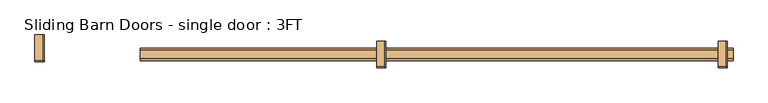
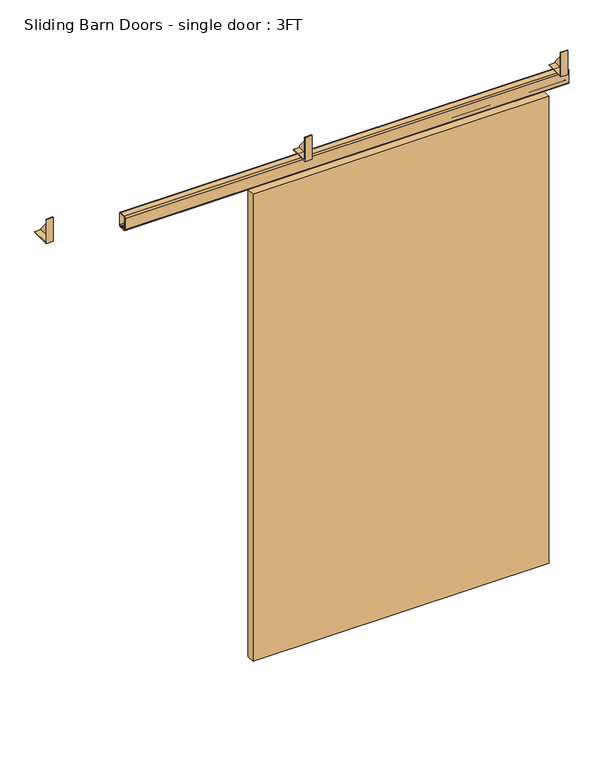
"""IFC4 building model written with IfcOpenShell, lengths in millimetres: door geometry, Sliding Barn Doors - single door : 3FT."""

from ifc_helpers import new_model, si_unit, point, frame, frame_2d, origin, place, context, project, spatial, polyline, circle_curve, trimmed, segment, composite_curve, outline, extrude, source, transform, mapped, element, save


def sliding_barn_doors_single_door_3ft_23110fb7(model_context):
    return source(origin(), model_context, "Body", "SweptSolid", [
        extrude(outline(polyline([(158.75, 2152.65), (158.75, 2146.3), (79.375, 2146.3), (79.375, 2247.773), (158.75, 2152.65)])), frame((-1538.3371094, 0.0, 0.0), z_axis=(1.0, 0.0, 0.0), x_axis=(0.0, 1.0, 0.0)), (0.0, 0.0, 1.0), 3.175),
        extrude(outline(polyline([(76.2, 2143.125), (76.2, 2247.773), (79.375, 2247.773), (79.375, 2146.3), (158.75, 2146.3), (158.75, 2143.125), (76.2, 2143.125)])), frame((-1563.6378906, 0.0, 0.0), z_axis=(1.0, 0.0, 0.0), x_axis=(0.0, 1.0, 0.0)), (0.0, 0.0, 1.0), 28.4757812),
        extrude(outline(polyline([(139.7, 2152.65), (139.7, 2146.3), (60.325, 2146.3), (60.325, 2247.773), (139.7, 2152.65)])), frame((-484.2371094, 0.0, 0.0), z_axis=(1.0, 0.0, 0.0), x_axis=(0.0, 1.0, 0.0)), (0.0, 0.0, 1.0), 3.175),
        extrude(outline(polyline([(57.15, 2143.125), (57.15, 2247.773), (60.325, 2247.773), (60.325, 2146.3), (139.7, 2146.3), (139.7, 2143.125), (57.15, 2143.125)])), frame((-509.5378906, 0.0, 0.0), z_axis=(1.0, 0.0, 0.0), x_axis=(0.0, 1.0, 0.0)), (0.0, 0.0, 1.0), 28.4757813),
        extrude(outline(polyline([(139.7, 2152.65), (139.7, 2146.3), (60.325, 2146.3), (60.325, 2247.773), (139.7, 2152.65)])), frame((569.8628906, 0.0, 0.0), z_axis=(1.0, 0.0, 0.0), x_axis=(0.0, 1.0, 0.0)), (0.0, 0.0, 1.0), 3.175),
        extrude(outline(polyline([(57.15, 2143.125), (57.15, 2247.773), (60.325, 2247.773), (60.325, 2146.3), (139.7, 2146.3), (139.7, 2143.125), (57.15, 2143.125)])), frame((544.5621094, 0.0, 0.0), z_axis=(1.0, 0.0, 0.0), x_axis=(0.0, 1.0, 0.0)), (0.0, 0.0, 1.0), 28.4757813),
        extrude(outline(polyline([(-609.854, 117.475), (-558.546, 117.475), (-558.546, 114.3), (-609.854, 114.3), (-609.854, 117.475)])), frame((0.0, 0.0, 1889.252), z_axis=(0.0, 0.0, 1.0), x_axis=(1.0, 0.0, 0.0)), (0.0, 0.0, 1.0), 168.148),
        extrude(outline(polyline([(355.346, 117.475), (406.654, 117.475), (406.654, 114.3), (355.346, 114.3), (355.346, 117.475)])), frame((0.0, 0.0, 1889.252), z_axis=(0.0, 0.0, 1.0), x_axis=(1.0, 0.0, 0.0)), (0.0, 0.0, 1.0), 168.148),
        extrude(outline(polyline([(-711.2, 114.3), (508.0, 114.3), (508.0, 79.375), (-711.2, 79.375), (-711.2, 114.3)])), frame((0.0, 0.0, 25.4), z_axis=(0.0, 0.0, 1.0), x_axis=(1.0, 0.0, 0.0)), (0.0, 0.0, 1.0), 2032.0),
        extrude(outline(composite_curve([segment(polyline([(85.725, 2143.125), (111.252, 2143.125)]), True, "CONTINUOUS"), segment(trimmed(circle_curve(frame_2d((111.252, 2136.775)), 6.35), [point((111.252, 2143.125))], [point((117.602, 2136.775))], False, "CARTESIAN"), True, "CONTINUOUS"), segment(polyline([(117.602, 2136.775), (117.602, 2088.515)]), True, "CONTINUOUS"), segment(trimmed(circle_curve(frame_2d((111.252, 2088.515)), 6.35), [point((117.602, 2088.515))], [point((111.252, 2082.165))], False, "CARTESIAN"), True, "CONTINUOUS"), segment(polyline([(111.252, 2082.165), (105.8433147, 2082.165)]), True, "CONTINUOUS"), segment(trimmed(circle_curve(frame_2d((105.8433147, 2083.7525)), 1.5875), [point((105.8433147, 2082.165))], [point((104.2849816, 2083.4495907))], False, "CARTESIAN"), True, "CONTINUOUS"), segment(polyline([(104.2849816, 2083.4495907), (102.8594659, 2090.7832331), (104.3756029, 2090.7832331), (105.7615251, 2083.6532812), (111.252, 2083.6532812)]), True, "CONTINUOUS"), segment(trimmed(circle_curve(frame_2d((111.252, 2088.515)), 4.8617187), [point((111.252, 2083.6532812))], [point((116.1137188, 2088.515))], True, "CARTESIAN"), True, "CONTINUOUS"), segment(polyline([(116.1137188, 2088.515), (116.1137188, 2136.775)]), True, "CONTINUOUS"), segment(trimmed(circle_curve(frame_2d((111.252, 2136.775)), 4.8617187), [point((116.1137188, 2136.775))], [point((111.252, 2141.6367187))], True, "CARTESIAN"), True, "CONTINUOUS"), segment(polyline([(111.252, 2141.6367187), (85.725, 2141.6367187)]), True, "CONTINUOUS"), segment(trimmed(circle_curve(frame_2d((85.725, 2136.775)), 4.8617187), [point((85.725, 2141.6367187))], [point((80.8632813, 2136.775))], True, "CARTESIAN"), True, "CONTINUOUS"), segment(polyline([(80.8632813, 2136.775), (80.8632813, 2088.515)]), True, "CONTINUOUS"), segment(trimmed(circle_curve(frame_2d((85.725, 2088.515)), 4.8617187), [point((80.8632813, 2088.515))], [point((85.725, 2083.6532812))], True, "CARTESIAN"), True, "CONTINUOUS"), segment(polyline([(85.725, 2083.6532812), (91.2154749, 2083.6532812), (92.6013971, 2090.7832331), (94.1175341, 2090.7832331), (92.6920184, 2083.4495907)]), True, "CONTINUOUS"), segment(trimmed(circle_curve(frame_2d((91.1336853, 2083.7525)), 1.5875), [point((92.6920184, 2083.4495907))], [point((91.1336853, 2082.165))], False, "CARTESIAN"), True, "CONTINUOUS"), segment(polyline([(91.1336853, 2082.165), (85.725, 2082.165)]), True, "CONTINUOUS"), segment(trimmed(circle_curve(frame_2d((85.725, 2088.515)), 6.35), [point((85.725, 2082.165))], [point((79.375, 2088.515))], False, "CARTESIAN"), True, "CONTINUOUS"), segment(polyline([(79.375, 2088.515), (79.375, 2136.775)]), True, "CONTINUOUS"), segment(trimmed(circle_curve(frame_2d((85.725, 2136.775)), 6.35), [point((79.375, 2136.775))], [point((85.725, 2143.125))], False, "CARTESIAN"), True, "CONTINUOUS")], self_intersect=False)), frame((-1238.25, 0.0, 0.0), z_axis=(1.0, 0.0, 0.0), x_axis=(0.0, 1.0, 0.0)), (0.0, 0.0, 1.0), 1828.8),
    ])


if __name__ == "__main__":
    model = new_model("IFC4")
    model_context = context("Model", 3, world=origin())
    ifc_project = project(units=[si_unit("LENGTHUNIT", "METRE", prefix="MILLI")], contexts=[model_context])
    site = spatial("IfcSite", under=ifc_project)
    building = spatial("IfcBuilding", under=site)
    placement = place(None, origin())
    sliding_barn_doors_single_door_3ft_shape = sliding_barn_doors_single_door_3ft_23110fb7(model_context)
    element("IfcDoor", 1, ObjectType="Sliding Barn Doors - single door : 3FT", at=placement, inside=building, context=model_context, shape_type="MappedRepresentation", body=[
        mapped(sliding_barn_doors_single_door_3ft_shape, transform((0.0, 0.0, 0.0), x_axis=(1.0, 0.0, 0.0), y_axis=(0.0, 1.0, 0.0), z_axis=(0.0, 0.0, 1.0))),
    ])
    save(model, "model.ifc")

# Revit data of these elements
# Type "Sliding Barn Doors - single door : 3FT"
#   Type Mark = "63"
#   Analytic Construction = "<None>"
#   rail_overlap_left = 0' - 5 1/4"
#   rail_length = 6' - 0"
#   overlap_left = 0' - 2"
#   overlap = 0' - 0"
#   bracket_right = 3' - 7"
#   bracket_left = 0' - 4"
#   Thickness = 0' - 1 3/8"
#   Panel Width = 4' - 0"
#   Panel Height = 6' - 8"
#   Gap 2 = 0' - 0 1/2"
#   Gap 1 = 0' - 0 7/8"
#   Frame Projection Ext. = 0' - 1"
#   Frame Projection Int. = 0' - 1"
#   Frame Width = 0' - 3"
#   Height = 6' - 4"
#   Width = 3' - 0"
#   Bracket_offset = 0' - 5"
#   Door_4 = no
#   Door_3 = no
#   Hardware Material = Metal - Aluminum
#   Door Material = Closet_1
#   Function = (empty or 0)
#   Wall Closure = (empty or 0)
# Element 1 (IfcDoor, "Sliding Barn Doors - single door : 3FT")
#   Materials on its faces: "Metal - Aluminum", "Closet_1"
# Materials
#   "Metal - Aluminum": class "Metal", colour RGB 247 247 247, transparency 0
#   "Closet_1": class "Paint", colour RGB 58 62 47, transparency 0, Cost = 0
